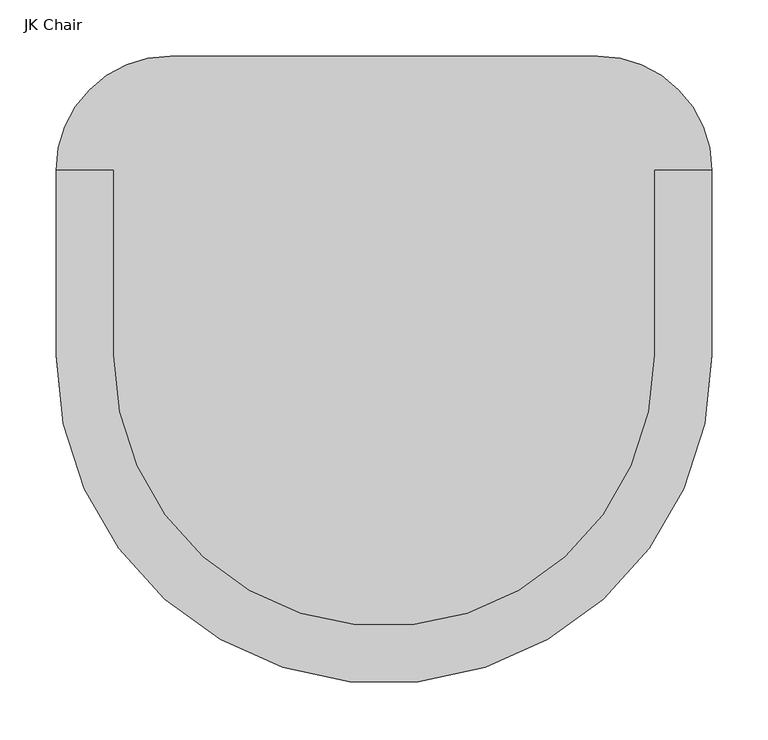
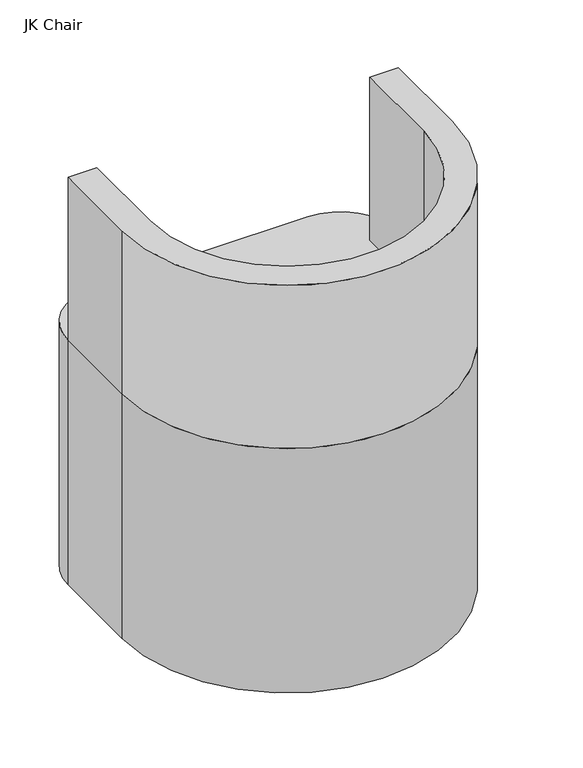
"""IFC4 building model written with IfcOpenShell, lengths in millimetres: furniture geometry, JK Chair : Recpt Chair."""

from ifc_helpers import new_model, si_unit, point, frame, frame_2d, origin, origin_with_axes, place, context, project, spatial, polyline, circle_curve, trimmed, segment, composite_curve, outline, extrude, source, transform, mapped, element, save


def jk_chair_074037dd(model_context):
    return source(origin(), model_context, "Body", "SweptSolid", [
        extrude(outline(composite_curve([segment(polyline([(-303.2426335, 131.5544704), (-303.2426335, -33.5455296)]), True, "CONTINUOUS"), segment(trimmed(circle_curve(frame_2d((-61.9426335, -33.5455296)), 241.3), [point((-303.2426335, -33.5455296))], [point((179.3573665, -33.5455296))], True, "CARTESIAN"), True, "CONTINUOUS"), segment(polyline([(179.3573665, -33.5455296), (179.3573665, 131.5544704), (230.1573665, 131.5544704), (230.1573665, -33.5455296)]), True, "CONTINUOUS"), segment(trimmed(circle_curve(frame_2d((-61.9426335, -33.5455296)), 292.1), [point((230.1573665, -33.5455296))], [point((-354.0426335, -33.5455296))], False, "CARTESIAN"), True, "CONTINUOUS"), segment(polyline([(-354.0426335, -33.5455296), (-354.0426335, 131.5544704), (-303.2426335, 131.5544704)]), True, "CONTINUOUS")], self_intersect=False)), frame((0.0, 0.0, 457.2), z_axis=(0.0, 0.0, 1.0), x_axis=(1.0, 0.0, 0.0)), (0.0, 0.0, 1.0), 304.8),
        extrude(outline(composite_curve([segment(polyline([(-354.0426335, -33.5455296), (-354.0426335, 131.5544704)]), True, "CONTINUOUS"), segment(trimmed(circle_curve(frame_2d((-252.4426335, 131.5544704)), 101.6), [point((-354.0426335, 131.5544704))], [point((-252.4426335, 233.1544704))], False, "CARTESIAN"), True, "CONTINUOUS"), segment(polyline([(-252.4426335, 233.1544704), (128.5573665, 233.1544704)]), True, "CONTINUOUS"), segment(trimmed(circle_curve(frame_2d((128.5573665, 131.5544704)), 101.6), [point((128.5573665, 233.1544704))], [point((230.1573665, 131.5544704))], False, "CARTESIAN"), True, "CONTINUOUS"), segment(polyline([(230.1573665, 131.5544704), (230.1573665, -33.5455296)]), True, "CONTINUOUS"), segment(trimmed(circle_curve(frame_2d((-61.9426335, -33.5455296)), 292.1), [point((230.1573665, -33.5455296))], [point((-354.0426335, -33.5455296))], False, "CARTESIAN"), True, "CONTINUOUS")], self_intersect=False)), origin_with_axes(), (0.0, 0.0, 1.0), 457.2),
    ])


if __name__ == "__main__":
    model = new_model("IFC4")
    model_context = context("Model", 3, world=origin())
    ifc_project = project(units=[si_unit("LENGTHUNIT", "METRE", prefix="MILLI")], contexts=[model_context])
    site = spatial("IfcSite", under=ifc_project)
    building = spatial("IfcBuilding", under=site)
    placement = place(None, origin())
    jk_chair_shape = jk_chair_074037dd(model_context)
    element("IfcFurniture", 1, ObjectType="JK Chair : Recpt Chair", at=placement, inside=building, context=model_context, shape_type="MappedRepresentation", body=[
        mapped(jk_chair_shape, transform((0.0, 0.0, 0.0), x_axis=(1.0, 0.0, 0.0), y_axis=(0.0, 1.0, 0.0), z_axis=(0.0, 0.0, 1.0))),
    ])
    save(model, "model.ifc")

# Revit data of these elements
# Type "JK Chair : Recpt Chair"
#   Width = 1' - 11"
#   Seat Height = 1' - 6"
#   Depth = 1' - 9"
#   Corner Radius = 0' - 4"
#   Back Height = 2' - 6"
#   Status [instance default] = none
#   Default Elevation = 0
